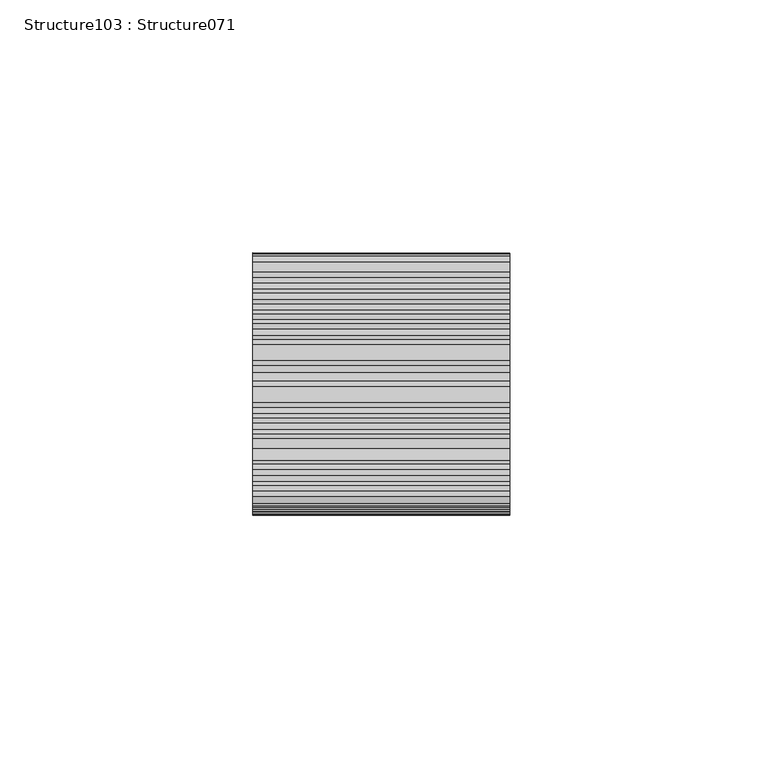
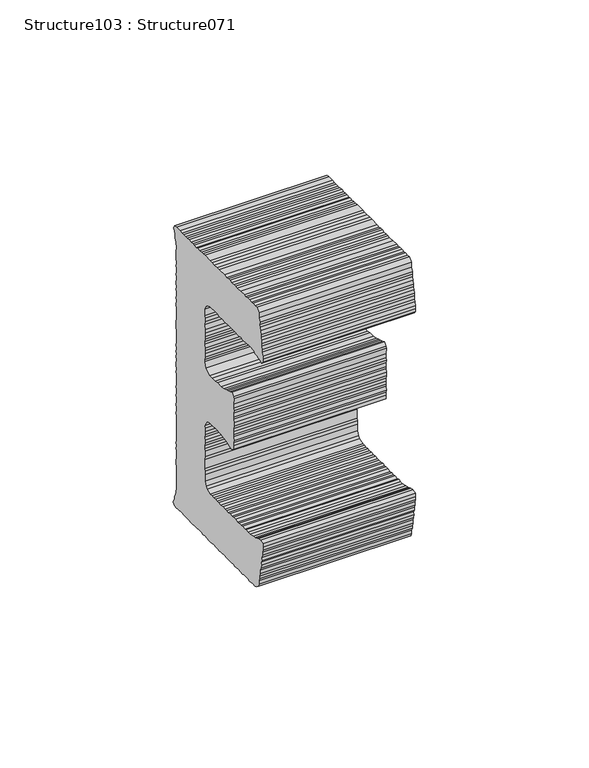
"""IFC4 building model written with IfcOpenShell, lengths in millimetres: proxy geometry, Structure103 : Structure071."""

from ifc_helpers import new_model, si_unit, frame, origin, place, context, project, spatial, polyline, outline, extrude, source, transform, mapped, element, save


def structure103_structure071_549b3acb(model_context):
    return source(origin(), model_context, "Body", "SweptSolid", [
        extrude(outline(polyline([(1.478812, 0.0), (2.2548681, -0.2742081), (3.0967006, -1.0995396), (4.8950919, -2.1683396), (5.4509723, -2.9345501), (7.2984119, -4.3745159), (8.0716328, -4.6442584), (9.0174004, -5.5451874), (9.7579227, -6.2915538), (10.576263, -6.9293998), (11.4550037, -7.2813886), (12.1121944, -8.1265642), (13.0125621, -8.659171), (15.4720729, -10.5762089), (16.0060457, -11.1615825), (17.6469357, -12.4405557), (18.728297, -12.9504748), (19.3698533, -13.6142896), (20.1884741, -14.2523544), (21.0263777, -15.0746235), (21.7241249, -15.4493), (22.7273877, -16.0675207), (23.4404887, -16.6233392), (25.1267786, -18.2706346), (25.9258361, -18.7242762), (26.6624294, -19.4675802), (29.8389702, -21.943499), (30.8229501, -22.3775152), (31.641571, -23.01558), (32.3024099, -23.8635992), (33.0978191, -24.3143972), (33.8341318, -25.0574825), (34.9452586, -25.7543631), (35.5805417, -26.4187019), (37.2175027, -27.6946127), (38.2233904, -28.3094658), (39.0456596, -28.9503742), (38.9190121, -30.16626), (37.6061312, -30.7972524), (36.9441986, -31.4294484), (35.9171214, -32.1122281), (34.9685719, -32.6942587), (33.644042, -33.9676066), (32.9042294, -34.7078236), (32.2887285, -35.7064392), (31.6250375, -36.3489942), (30.3456269, -37.9904455), (29.8097474, -38.886909), (29.0699349, -39.6271259), (28.6390758, -40.6058976), (27.9187648, -41.5300383), (27.2570508, -42.1619537), (26.4330234, -43.0102162), (25.8175225, -44.0088319), (25.3601623, -44.8126602), (24.6177333, -45.548131), (24.0844703, -46.4493406), (23.3190398, -47.0053779), (22.7829416, -47.902122), (22.0650367, -48.8231757), (21.4024394, -49.4643275), (20.7639372, -50.2835096), (20.1484363, -51.2821253), (19.4062176, -52.0254292), (18.8690257, -52.9235766), (18.2064284, -53.5647284), (17.6950731, -54.6467747), (16.8730226, -55.4843977), (16.2887342, -56.0250812), (15.858094, -57.0035721), (14.9310147, -57.7670008), (14.3938228, -58.6651481), (13.7824695, -59.6665455), (13.0964418, -60.1207112), (12.4772224, -61.1240976), (12.0270805, -61.9186649), (11.0967201, -62.6863032), (10.5608406, -63.5827667), (9.2838362, -65.2211309), (8.6698581, -66.2258959), (7.9827366, -66.6814648), (7.3906661, -67.8670666), (6.8339727, -68.5812901), (6.0060163, -69.4264903), (5.473847, -70.3262968), (4.6327325, -70.9794348), (4.3560853, -71.7603567), (3.4314121, -72.5206983), (2.918963, -73.604148), (2.07413, -74.2620567), (0.7947194, -75.903508), (0.3369301, -76.6997838), (-0.3004784, -77.5175626), (-0.7541201, -78.3166202), (-2.1151207, -80.0627494), (-3.0384815, -80.8214072), (-4.134773, -82.4368651), (-4.9563943, -83.2820406), (-5.8678252, -84.8773738), (-6.6896569, -85.7147161), (-7.2251073, -86.6187322), (-8.0473765, -87.4566358), (-8.68566, -88.2755373), (-9.0636176, -88.977494), (-9.8073591, -89.7146487), (-10.3428095, -90.6186647), (-11.9829814, -92.296973), (-12.2572225, -93.0748079), (-13.1009618, -93.7313135), (-13.7980528, -94.8346072), (-14.1736041, -95.5334768), (-15.1006835, -96.2969055), (-15.6109451, -97.3775487), (-17.3696152, -99.6338777), (-18.2927572, -100.3922549), (-19.2079067, -101.9923589), (-19.4100899, -103.3126793), (-20.0258095, -104.3115756), (-20.4599496, -105.2945568), (-20.7148377, -106.2489816), (-21.57793, -106.7288973), (-22.5885596, -106.1126038), (-24.1244911, -104.9154394), (-24.9610203, -104.0919859), (-25.7796412, -103.4539211), (-26.7905515, -102.8374088), (-27.319221, -102.2539131), (-28.5058215, -101.6619665), (-29.0614213, -100.8959748), (-30.0684026, -100.2825249), (-30.6844028, -99.8023905), (-31.5209321, -98.9789369), (-32.2944336, -98.7089756), (-32.9552726, -97.8609564), (-34.1418732, -97.2690098), (-34.6795644, -96.688407), (-35.5762136, -96.1510294), (-38.0357245, -94.2339915), (-38.7760365, -93.4954582), (-39.7220145, -92.586696), (-41.134237, -91.6573855), (-42.1361254, -91.0379804), (-44.5956363, -89.1209425), (-45.2528269, -88.2757669), (-46.3381172, -87.7627854), (-47.0512182, -87.2069669), (-47.6110275, -86.4376941), (-48.6359172, -85.6388554), (-49.4324201, -85.1894606), (-50.0705383, -84.5206562), (-51.6061892, -83.3237106), (-53.6111299, -82.093918), (-54.0657, -81.4066727), (-55.0454705, -80.9759375), (-55.9693305, -80.2558452), (-56.8148817, -79.4352845), (-57.5049813, -79.0588996), (-58.3505324, -78.2383389), (-59.1691533, -77.6002741), (-59.552041, -75.977763), (-58.4340605, -74.5434226), (-58.0446725, -73.1993911), (-57.3844814, -72.5613264), (-57.0052197, -71.8657996), (-56.6798187, -70.8052811), (-56.0798904, -69.6258041), (-55.4194805, -68.9874587), (-55.0671491, -68.109436), (-54.6277676, -67.1278333), (-54.0723866, -66.4152937), (-53.4573148, -65.4091254), (-53.0789282, -64.7147213), (-52.6702575, -63.5548942), (-52.2128973, -62.7510659), (-51.5746138, -61.9321644), (-50.3958036, -61.6983312), (-50.208394, -62.5026078), (-49.3624138, -63.3307211), (-48.7020039, -64.1711877), (-47.9651918, -64.914211), (-47.7737912, -65.7220493), (-46.084282, -67.3646358), (-44.447321, -68.6405465), (-43.5681511, -69.0000879), (-42.6485005, -69.7168991), (-41.9838811, -70.5606468), (-41.0073299, -70.996091), (-40.2942289, -71.5519095), (-39.6296095, -72.3956572), (-38.5259114, -73.0939656), (-36.0664005, -75.0110035), (-35.1686577, -75.546978), (-34.4513471, -76.1060776), (-33.685698, -77.0285717), (-32.8104571, -77.3850507), (-31.8646894, -78.2859797), (-31.3314264, -78.8635821), (-29.6902558, -80.142774), (-28.7894589, -80.6829333), (-27.9480554, -81.5007123), (-26.2173558, -82.0295278), (-25.0431843, -81.784861), (-23.7331556, -81.1656307), (-22.2960333, -79.3218394), (-21.9167717, -78.6263128), (-21.3014895, -77.6279778), (-20.3761518, -76.8586803), (-19.4377905, -75.4458431), (-18.7207606, -74.525912), (-18.1054785, -73.5275769), (-17.5426603, -72.8054955), (-16.7030687, -72.1462081), (-16.1463752, -71.4319845), (-15.6262786, -70.3468265), (-15.0708976, -69.6342868), (-14.2492762, -68.7891113), (-13.7120843, -67.890964), (-12.8720552, -67.2311153), (-12.3892959, -66.6117474), (-11.706384, -64.6740854), (-12.8293732, -62.3208744), (-13.7725161, -61.4165777), (-15.2068566, -60.2985973), (-16.3962924, -59.7021851), (-18.0332535, -58.4262743), (-19.7084267, -57.6172762), (-20.9733362, -57.1257979), (-21.8480777, -56.769257), (-22.9294391, -56.259338), (-24.0700369, -56.0262584), (-24.3270901, -54.6682954), (-23.9550385, -53.9739159), (-22.4692971, -52.4937379), (-21.7743936, -51.3932507), (-21.396436, -50.691294), (-20.5553215, -50.038156), (-19.8577932, -48.9343011), (-19.2772233, -48.3983885), (-18.7630244, -47.3126939), (-18.046432, -46.393324), (-17.1989741, -45.7320476), (-16.5606905, -44.913146), (-16.0994014, -44.1123801), (-15.4427101, -43.4788056), (-14.9324484, -42.3981623), (-14.1632994, -41.8373542), (-13.62742, -40.9408908), (-12.9095151, -40.0198371), (-11.4055762, -40.1959649), (-11.0069783, -41.1720678), (-10.4502848, -41.9366562), (-9.5843488, -42.9319043), (-9.0052567, -43.8853815), (-7.7054161, -45.3929685), (-6.910007, -45.8437665), (-5.9671447, -46.7478445), (-5.4305472, -47.3298505), (-4.2439466, -47.9217971), (-3.6128731, -48.5828549), (-2.6850841, -49.3060095), (-0.9508846, -49.8303349), (1.4256702, -48.8874973), (1.7060278, -48.1099184), (2.6024582, -47.1687647), (3.2409604, -46.3495826), (3.9048701, -45.7067469), (4.2576306, -44.8362769), (4.8983202, -44.0142884), (5.8212518, -43.248078), (6.459754, -42.4288958), (6.837922, -41.7347723), (8.0353051, -40.1985603), (8.8558327, -39.3547879), (10.7735268, -36.8944351), (11.1516948, -36.2003116), (11.7671956, -35.201696), (13.1260089, -33.4583731), (13.6726794, -31.9044491), (13.7445103, -30.9765171), (12.5266972, -29.3636907), (11.6260488, -28.8308651), (11.1717593, -28.1438387), (9.9851588, -27.551892), (9.5305887, -26.8646468), (8.6328458, -26.3286723), (7.7923173, -25.5097708), (6.6017878, -24.9147618), (5.9448777, -24.069805), (5.0468543, -23.5336118), (4.4089463, -22.8726407), (3.3239368, -22.3598779), (2.7680563, -21.5936675), (1.9716238, -21.1366582), (0.9696651, -20.5248675), (0.101996, -19.5156369), (-0.6944366, -19.0586276), (-1.4297259, -18.3217537), (-2.3123955, -17.9667025), (-3.1758551, -16.960753), (-3.9532856, -16.6877293), (-4.6101956, -15.8427726), (-5.4288164, -15.2047078), (-7.3923481, -14.3396756), (-8.2894966, -13.8023598), (-9.1680186, -13.4500903), (-10.1226003, -13.1959823), (-11.3118173, -12.5992895), (-12.2781803, -11.5158399), (-11.4782478, -10.489547), (-10.8408393, -9.671768), (-10.1537179, -9.2161992), (-9.253507, -8.270774), (-8.3032159, -7.694612), (-7.8495743, -6.8955546), (-6.8773756, -6.5002294), (-6.3419252, -5.5962134), (-5.4185646, -4.8375555), (-4.5555341, -4.3571405), (-3.7569141, -3.3325314), (-2.9914837, -2.7764942), (-2.4326028, -2.0594642), (-1.483554, -1.4773716), (-0.5858112, -0.5345341), (0.0, 0.0), (1.478812, 0.0)])), frame((-56111.5333239, 291240.3769088, -374.3014721), z_axis=(-0.9999998917542983, 0.00046528635450596156, 0.0), x_axis=(0.00036697923779000164, 0.7887168718991745, -0.614756505705975)), (0.0, 0.0, 1.0), 50.8),
    ])


if __name__ == "__main__":
    model = new_model("IFC4")
    model_context = context("Model", 3, world=origin())
    ifc_project = project(units=[si_unit("LENGTHUNIT", "METRE", prefix="MILLI")], contexts=[model_context])
    site = spatial("IfcSite", under=ifc_project)
    building = spatial("IfcBuilding", under=site)
    placement = place(None, origin())
    structure103_structure071_shape = structure103_structure071_549b3acb(model_context)
    element("IfcBuildingElementProxy", 1, Name="Structure103 : Structure071", ObjectType="Structure103 : Structure071", at=placement, inside=building, context=model_context, shape_type="MappedRepresentation", body=[
        mapped(structure103_structure071_shape, transform((0.0, 0.0, 0.0), x_axis=(1.0, 0.0, 0.0), y_axis=(0.0, 1.0, 0.0), z_axis=(0.0, 0.0, 1.0))),
    ])
    save(model, "model.ifc")

# Revit data of these elements
# Type "Structure103 : Structure071"
#   NameOverride = "Structure071"
# Element 1 (IfcBuildingElementProxy, "Structure103 : Structure071")
#   Materials on its faces: "BRUSHED ALUMINUM LETTERING"
# Materials
#   "BRUSHED ALUMINUM LETTERING": class "Unassigned", colour RGB 169 181 186, transparency 0, Cost = 0
